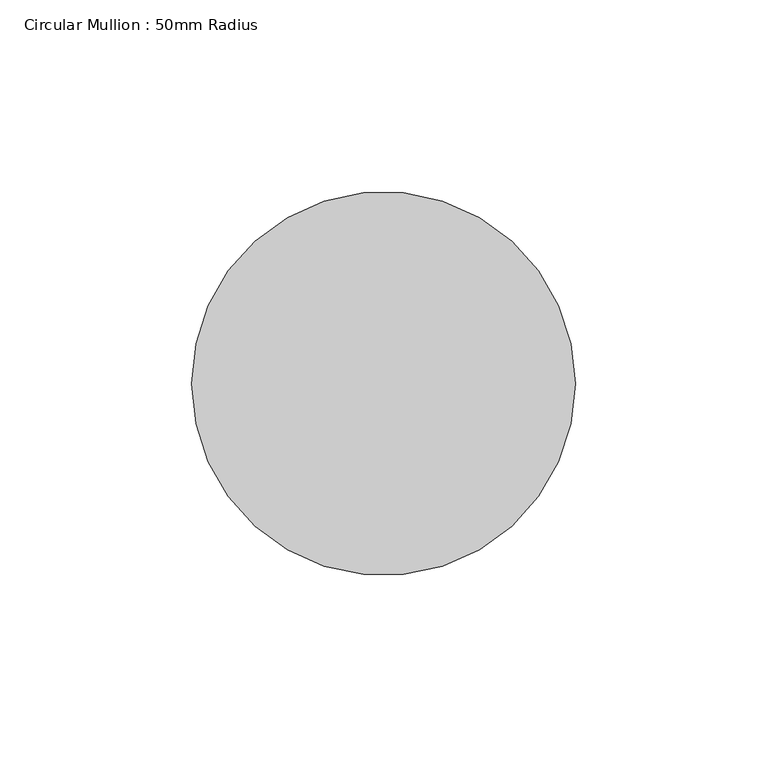
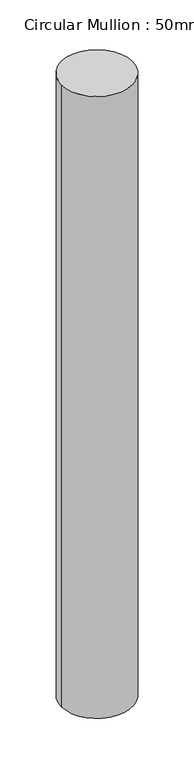
"""IFC4 building model written with IfcOpenShell, lengths in millimetres: member geometry, Circular Mullion : 50mm Radius."""

from ifc_helpers import new_model, si_unit, point, frame, origin, origin_2d, place, context, project, spatial, circle_curve, trimmed, segment, composite_curve, outline, extrude, source, transform, mapped, element, save


def circular_mullion_50mm_radius_a76fa9c7(model_context):
    return source(origin(), model_context, "Body", "SweptSolid", [
        extrude(outline(composite_curve([segment(trimmed(circle_curve(origin_2d(), 50.0), [point((50.0, 0.0))], [point((-50.0, 0.0))], False, "CARTESIAN"), True, "CONTINUOUS"), segment(trimmed(circle_curve(origin_2d(), 50.0), [point((-50.0, 0.0))], [point((50.0, 0.0))], False, "CARTESIAN"), True, "CONTINUOUS")], self_intersect=False)), frame((0.0, 0.0, -927.1232857), z_axis=(0.0, 0.0, 1.0), x_axis=(1.0, 0.0, 0.0)), (0.0, 0.0, 1.0), 927.1232857),
    ])


if __name__ == "__main__":
    model = new_model("IFC4")
    model_context = context("Model", 3, world=origin())
    ifc_project = project(units=[si_unit("LENGTHUNIT", "METRE", prefix="MILLI")], contexts=[model_context])
    site = spatial("IfcSite", under=ifc_project)
    building = spatial("IfcBuilding", under=site)
    placement = place(None, origin())
    circular_mullion_50mm_radius_shape = circular_mullion_50mm_radius_a76fa9c7(model_context)
    element("IfcMember", 1, ObjectType="Circular Mullion : 50mm Radius", at=placement, inside=building, context=model_context, shape_type="MappedRepresentation", body=[
        mapped(circular_mullion_50mm_radius_shape, transform((0.0, 0.0, 0.0), x_axis=(1.0, 0.0, 0.0), y_axis=(0.0, 1.0, 0.0), z_axis=(0.0, 0.0, 1.0))),
    ])
    save(model, "model.ifc")

# Revit data of these elements
# Type "Circular Mullion : 50mm Radius"
#   built-in parameter 1007350 = 0.164042 (stored number, unit not read)
# Element 1 (IfcMember, "Circular Mullion : 50mm Radius")
#   Materials on its faces: "Aluminium"
# Materials
#   "Aluminium": class "Metal", colour RGB 247 247 247, transparency 0, Description = "Aluminium 6061", Cost = 0
